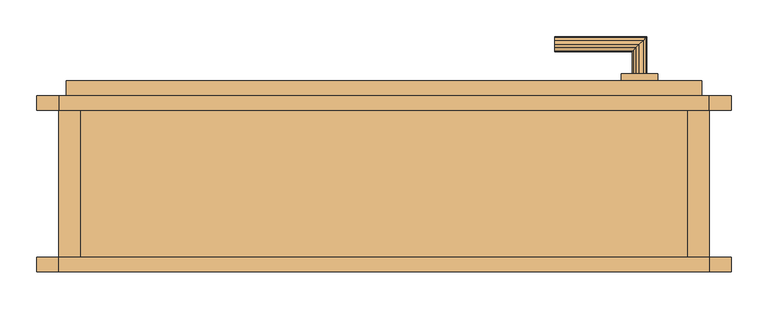
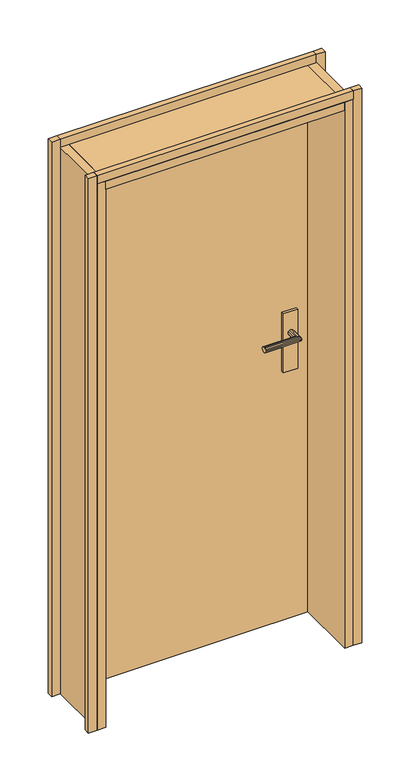
"""IFC4 building model written with IfcOpenShell, lengths in millimetres: door geometry, Tür."""

from ifc_helpers import new_model, si_unit, frame, origin, place, context, project, spatial, polyline, outline, extrude, faceted_brep, source, transform, mapped, element, save


def door_fcbd9d32(model_context):
    return source(origin(), model_context, "Body", "SolidModel", [
        extrude(outline(polyline([(0.0, 200.0), (-30.0, 200.0), (-30.0, 220.0), (0.0, 220.0), (0.0, 200.0)])), frame((0.0, 0.0, 140.0), z_axis=(0.0, 0.0, 1.0), x_axis=(1.0, 0.0, 0.0)), (0.0, 0.0, 1.0), 2025.0),
        extrude(outline(polyline([(855.0, 220.0), (855.0, -20.0), (30.0, -20.0), (30.0, 220.0), (855.0, 220.0)])), frame((0.0, 0.0, 2105.0), z_axis=(0.0, 0.0, 1.0), x_axis=(1.0, 0.0, 0.0)), (0.0, 0.0, 1.0), 30.0),
        extrude(outline(polyline([(885.0, 0.0), (885.0, -20.0), (0.0, -20.0), (0.0, 0.0), (885.0, 0.0)])), frame((0.0, 0.0, 2135.0), z_axis=(0.0, 0.0, 1.0), x_axis=(1.0, 0.0, 0.0)), (0.0, 0.0, 1.0), 30.0),
        extrude(outline(polyline([(915.0, 0.0), (915.0, -20.0), (885.0, -20.0), (885.0, 0.0), (915.0, 0.0)])), frame((0.0, 0.0, 140.0), z_axis=(0.0, 0.0, 1.0), x_axis=(1.0, 0.0, 0.0)), (0.0, 0.0, 1.0), 2025.0),
        extrude(outline(polyline([(30.0, 220.0), (30.0, -20.0), (0.0, -20.0), (0.0, 220.0), (30.0, 220.0)])), frame((0.0, 0.0, 140.0), z_axis=(0.0, 0.0, 1.0), x_axis=(1.0, 0.0, 0.0)), (0.0, 0.0, 1.0), 1995.0),
        extrude(outline(polyline([(765.0, 200.0), (815.0, 200.0), (815.0, 190.0), (765.0, 190.0), (765.0, 200.0)])), frame((0.0, 0.0, 1050.0), z_axis=(0.0, 0.0, 1.0), x_axis=(1.0, 0.0, 0.0)), (0.0, 0.0, 1.0), 215.0),
        faceted_brep([(785.0, 190.0, 1198.660254), (790.0, 190.0, 1200.0), (795.0, 190.0, 1198.660254), (798.660254, 190.0, 1195.0), (800.0, 190.0, 1190.0), (798.660254, 190.0, 1185.0), (795.0, 190.0, 1181.339746), (790.0, 190.0, 1180.0), (785.0, 190.0, 1181.339746), (781.339746, 190.0, 1185.0), (780.0, 190.0, 1190.0), (781.339746, 190.0, 1195.0), (790.0, 150.0, 1200.0), (795.0, 145.0, 1198.660254), (798.660254, 141.339746, 1195.0), (800.0, 140.0, 1190.0), (798.660254, 141.339746, 1185.0), (795.0, 145.0, 1181.339746), (790.0, 150.0, 1180.0), (785.0, 155.0, 1181.339746), (781.339746, 158.660254, 1185.0), (780.0, 160.0, 1190.0), (781.339746, 158.660254, 1195.0), (785.0, 155.0, 1198.660254), (675.0, 145.0, 1198.660254), (675.0, 150.0, 1200.0), (675.0, 155.0, 1198.660254), (675.0, 158.660254, 1195.0), (675.0, 160.0, 1190.0), (675.0, 158.660254, 1185.0), (675.0, 155.0, 1181.339746), (675.0, 150.0, 1180.0), (675.0, 145.0, 1181.339746), (675.0, 141.339746, 1185.0), (675.0, 140.0, 1190.0), (675.0, 141.339746, 1195.0)], [[[0, 1, 2, 3, 4, 5, 6, 7, 8, 9, 10, 11]], [[2, 1, 12, 13]], [[3, 2, 13, 14]], [[4, 3, 14, 15]], [[5, 4, 15, 16]], [[6, 5, 16, 17]], [[7, 6, 17, 18]], [[8, 7, 18, 19]], [[9, 8, 19, 20]], [[10, 9, 20, 21]], [[11, 10, 21, 22]], [[0, 11, 22, 23]], [[1, 0, 23, 12]], [[24, 25, 26, 27, 28, 29, 30, 31, 32, 33, 34, 35]], [[13, 12, 25, 24]], [[14, 13, 24, 35]], [[15, 14, 35, 34]], [[16, 15, 34, 33]], [[17, 16, 33, 32]], [[18, 17, 32, 31]], [[19, 18, 31, 30]], [[20, 19, 30, 29]], [[21, 20, 29, 28]], [[22, 21, 28, 27]], [[23, 22, 27, 26]], [[12, 23, 26, 25]]]),
        extrude(outline(polyline([(885.0, 220.0), (885.0, -20.0), (855.0, -20.0), (855.0, 220.0), (885.0, 220.0)])), frame((0.0, 0.0, 140.0), z_axis=(0.0, 0.0, 1.0), x_axis=(1.0, 0.0, 0.0)), (0.0, 0.0, 1.0), 1995.0),
        faceted_brep([(795.0, 250.0, 1198.660254), (790.0, 250.0, 1200.0), (785.0, 250.0, 1198.660254), (781.339746, 250.0, 1195.0), (780.0, 250.0, 1190.0), (781.339746, 250.0, 1185.0), (785.0, 250.0, 1181.339746), (790.0, 250.0, 1180.0), (795.0, 250.0, 1181.339746), (798.660254, 250.0, 1185.0), (800.0, 250.0, 1190.0), (798.660254, 250.0, 1195.0), (790.0, 290.0, 1200.0), (795.0, 295.0, 1198.660254), (798.660254, 298.660254, 1195.0), (800.0, 300.0, 1190.0), (798.660254, 298.660254, 1185.0), (795.0, 295.0, 1181.339746), (790.0, 290.0, 1180.0), (785.0, 285.0, 1181.339746), (781.339746, 281.339746, 1185.0), (780.0, 280.0, 1190.0), (781.339746, 281.339746, 1195.0), (785.0, 285.0, 1198.660254), (675.0, 285.0, 1198.660254), (675.0, 290.0, 1200.0), (675.0, 295.0, 1198.660254), (675.0, 298.660254, 1195.0), (675.0, 300.0, 1190.0), (675.0, 298.660254, 1185.0), (675.0, 295.0, 1181.339746), (675.0, 290.0, 1180.0), (675.0, 285.0, 1181.339746), (675.0, 281.339746, 1185.0), (675.0, 280.0, 1190.0), (675.0, 281.339746, 1195.0)], [[[0, 1, 2, 3, 4, 5, 6, 7, 8, 9, 10, 11]], [[12, 1, 0, 13]], [[13, 0, 11, 14]], [[14, 11, 10, 15]], [[15, 10, 9, 16]], [[16, 9, 8, 17]], [[17, 8, 7, 18]], [[18, 7, 6, 19]], [[19, 6, 5, 20]], [[20, 5, 4, 21]], [[21, 4, 3, 22]], [[22, 3, 2, 23]], [[23, 2, 1, 12]], [[24, 25, 26, 27, 28, 29, 30, 31, 32, 33, 34, 35]], [[25, 12, 13, 26]], [[26, 13, 14, 27]], [[27, 14, 15, 28]], [[28, 15, 16, 29]], [[29, 16, 17, 30]], [[30, 17, 18, 31]], [[31, 18, 19, 32]], [[32, 19, 20, 33]], [[33, 20, 21, 34]], [[34, 21, 22, 35]], [[35, 22, 23, 24]], [[24, 23, 12, 25]]]),
        extrude(outline(polyline([(915.0, 220.0), (915.0, 200.0), (885.0, 200.0), (885.0, 220.0), (915.0, 220.0)])), frame((0.0, 0.0, 140.0), z_axis=(0.0, 0.0, 1.0), x_axis=(1.0, 0.0, 0.0)), (0.0, 0.0, 1.0), 2025.0),
        extrude(outline(polyline([(885.0, 220.0), (885.0, 200.0), (0.0, 200.0), (0.0, 220.0), (885.0, 220.0)])), frame((0.0, 0.0, 2135.0), z_axis=(0.0, 0.0, 1.0), x_axis=(1.0, 0.0, 0.0)), (0.0, 0.0, 1.0), 30.0),
        extrude(outline(polyline([(815.0, 250.0), (815.0, 240.0), (765.0, 240.0), (765.0, 250.0), (815.0, 250.0)])), frame((0.0, 0.0, 1050.0), z_axis=(0.0, 0.0, 1.0), x_axis=(1.0, 0.0, 0.0)), (0.0, 0.0, 1.0), 215.0),
        extrude(outline(polyline([(0.0, -20.0), (-30.0, -20.0), (-30.0, 0.0), (0.0, 0.0), (0.0, -20.0)])), frame((0.0, 0.0, 140.0), z_axis=(0.0, 0.0, 1.0), x_axis=(1.0, 0.0, 0.0)), (0.0, 0.0, 1.0), 2025.0),
        extrude(outline(polyline([(875.0, 240.0), (875.0, 200.0), (10.0, 200.0), (10.0, 240.0), (875.0, 240.0)])), frame((0.0, 0.0, 140.0), z_axis=(0.0, 0.0, 1.0), x_axis=(1.0, 0.0, 0.0)), (0.0, 0.0, 1.0), 1985.0),
    ])


if __name__ == "__main__":
    model = new_model("IFC4")
    model_context = context("Model", 3, world=origin())
    ifc_project = project(units=[si_unit("LENGTHUNIT", "METRE", prefix="MILLI")], contexts=[model_context])
    site = spatial("IfcSite", under=ifc_project)
    building = spatial("IfcBuilding", under=site)
    placement = place(None, origin())
    door_shape = door_fcbd9d32(model_context)
    element("IfcDoor", 1, ObjectType="Tür", at=placement, inside=building, context=model_context, shape_type="MappedRepresentation", body=[
        mapped(door_shape, transform((0.0, 0.0, 0.0), x_axis=(1.0, 0.0, 0.0), y_axis=(0.0, 1.0, 0.0), z_axis=(0.0, 0.0, 1.0))),
    ])
    save(model, "model.ifc")

# Revit data of these elements
# Type "Tür"
#   Type Mark = "41"
# Element 1 (IfcDoor, "Tür")
#   Materials on its faces: "tuer_beschlag", "tuer_holzzarge"
# Materials
#   "tuer_beschlag": class "Unassigned", colour RGB 128 128 128, transparency 0
#   "tuer_holzzarge": class "Unassigned", colour RGB 255 255 255, transparency 0
